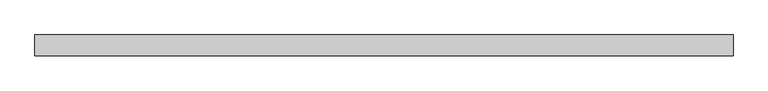
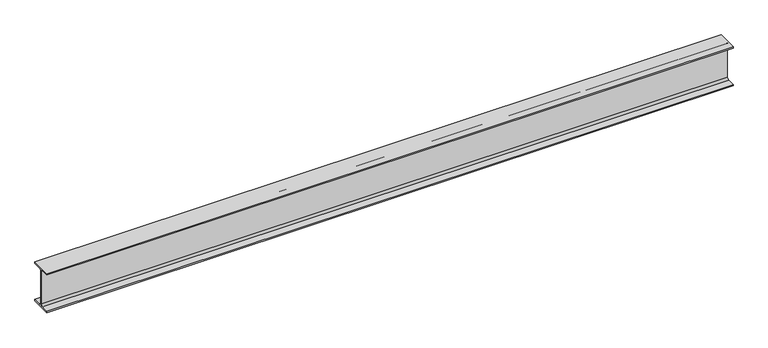
"""IFC4 building model written with IfcOpenShell, lengths in millimetres: beam geometry, 0912_Steel Framing_H-KSD3502 : H_SB_ASB_H-250x125x6x9."""

from ifc_helpers import new_model, si_unit, point, frame, frame_2d, origin, place, context, project, spatial, polyline, circle_curve, trimmed, segment, composite_curve, outline, extrude, source, transform, mapped, element, save


def beam_26006502(model_context):
    return source(origin(), model_context, "Body", "SweptSolid", [
        extrude(outline(composite_curve([segment(polyline([(62.5, -116.0), (62.5, -125.0), (-62.5, -125.0), (-62.5, -116.0), (-15.0, -116.0)]), True, "CONTINUOUS"), segment(trimmed(circle_curve(frame_2d((-15.0, -104.0)), 12.0), [point((-15.0, -116.0))], [point((-3.0, -104.0))], True, "CARTESIAN"), True, "CONTINUOUS"), segment(polyline([(-3.0, -104.0), (-3.0, 104.0)]), True, "CONTINUOUS"), segment(trimmed(circle_curve(frame_2d((-15.0, 104.0)), 12.0), [point((-3.0, 104.0))], [point((-15.0, 116.0))], True, "CARTESIAN"), True, "CONTINUOUS"), segment(polyline([(-15.0, 116.0), (-62.5, 116.0), (-62.5, 125.0), (62.5, 125.0), (62.5, 116.0), (15.0, 116.0)]), True, "CONTINUOUS"), segment(trimmed(circle_curve(frame_2d((15.0, 104.0)), 12.0), [point((15.0, 116.0))], [point((3.0, 104.0))], True, "CARTESIAN"), True, "CONTINUOUS"), segment(polyline([(3.0, 104.0), (3.0, -104.0)]), True, "CONTINUOUS"), segment(trimmed(circle_curve(frame_2d((15.0, -104.0)), 12.0), [point((3.0, -104.0))], [point((15.0, -116.0))], True, "CARTESIAN"), True, "CONTINUOUS"), segment(polyline([(15.0, -116.0), (62.5, -116.0)]), True, "CONTINUOUS")], self_intersect=False)), frame((-2112.2999994, 0.0, 0.0), z_axis=(1.0, 0.0, 0.0), x_axis=(0.0, 1.0, 0.0)), (0.0, 0.0, 1.0), 4142.0999994),
    ])


if __name__ == "__main__":
    model = new_model("IFC4")
    model_context = context("Model", 3, world=origin())
    ifc_project = project(units=[si_unit("LENGTHUNIT", "METRE", prefix="MILLI")], contexts=[model_context])
    site = spatial("IfcSite", under=ifc_project)
    building = spatial("IfcBuilding", under=site)
    placement = place(None, origin())
    beam_shape = beam_26006502(model_context)
    element("IfcBeam", 1, ObjectType="0912_Steel Framing_H-KSD3502 : H_SB_ASB_H-250x125x6x9", at=placement, inside=building, context=model_context, shape_type="MappedRepresentation", body=[
        mapped(beam_shape, transform((0.0, 0.0, 0.0), x_axis=(1.0, 0.0, 0.0), y_axis=(0.0, 1.0, 0.0), z_axis=(0.0, 0.0, 1.0))),
    ])
    save(model, "model.ifc")

# Revit data of these elements
# Type "0912_Steel Framing_H-KSD3502 : H_SB_ASB_H-250x125x6x9"
#   H_WM Code_1 = "S01AA003-00001 | Main Steel Structure Fabrication Work | Shelter/Building | Light Steel - Standard (30KG/M>Weight) | Material: (   )"
#   H_WM Code_2 = "S03AA029-00001 | Main Steel Structure Erection Work | Shelter/Building | Light Steel (30KG/M>Weight) | Material: (   )"
#   H_WM Code_3 = "S01AA010-00001 | Main Steel Structure Fabrication Work | Shelter/Building | Steel Painting/Coating | for Non-Fireproofed Steel Surface, Surface Preparation, Primer, Second & Final Coat | Material: (   )"
#   H_Q'ty Cal Type Tag = "SB-Q2"
#   Width = 12.5 cm
#   Web Thickness = 0.6 cm
#   Web Fillet = 1.2 cm
#   Warping Constant = 42539.8 cm⁶
#   W = 0
#   Torsional Moment of Inertia = 7.8102 cm⁴
#   Section Area = 37.66 cm²
#   Plastic Modulus weak axis = 73.1 cm³
#   Plastic Modulus strong axis = 366.0 cm³
#   Perimeter = 0.97 m²/m
#   Nominal Weight = 29.60 kgf/m
#   Moment of Inertia weak axis = 294.00 cm⁴
#   Moment of Inertia strong axis = 4050.00 cm⁴
#   Height = 25.0 cm
#   Flange Thickness = 0.9 cm
#   Elastic Modulus weak axis = 47.0 cm³
#   Elastic Modulus strong axis = 324.0 cm³
#   Centroid Vertical = 12.5 cm
#   Centroid Horizontal = 6.25 cm
#   Ix = 40500000
#   Length [instance default] = 1.5240 m
#   Zx = 366000
#   b = 0.1250 m
#   h = 0.2500 m
#   r = 0.0120 m
#   s = 0.0060 m
#   t = 0.0090 m
#   A = 0.003766 m²
#   Structural Material [instance default] = Steel, 45-345
#   Assembly Code = ""
# Element 1 (IfcBeam, "0912_Steel Framing_H-KSD3502 : H_SB_ASB_H-250x125x6x9")
#   Structural Material = none
# Materials
#   "Steel, 45-345": class "Metal", colour RGB 189 187 185, transparency 0, Description = "Steel 345 MPa", Cost = 0
